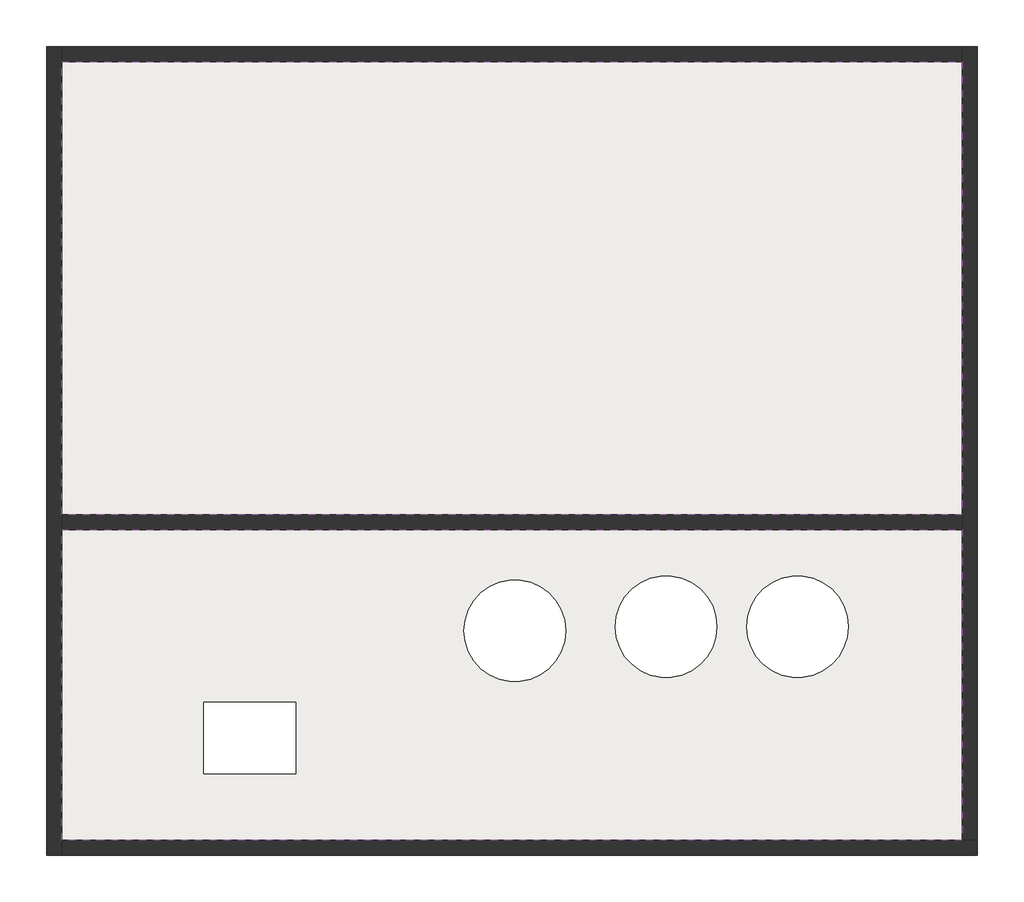
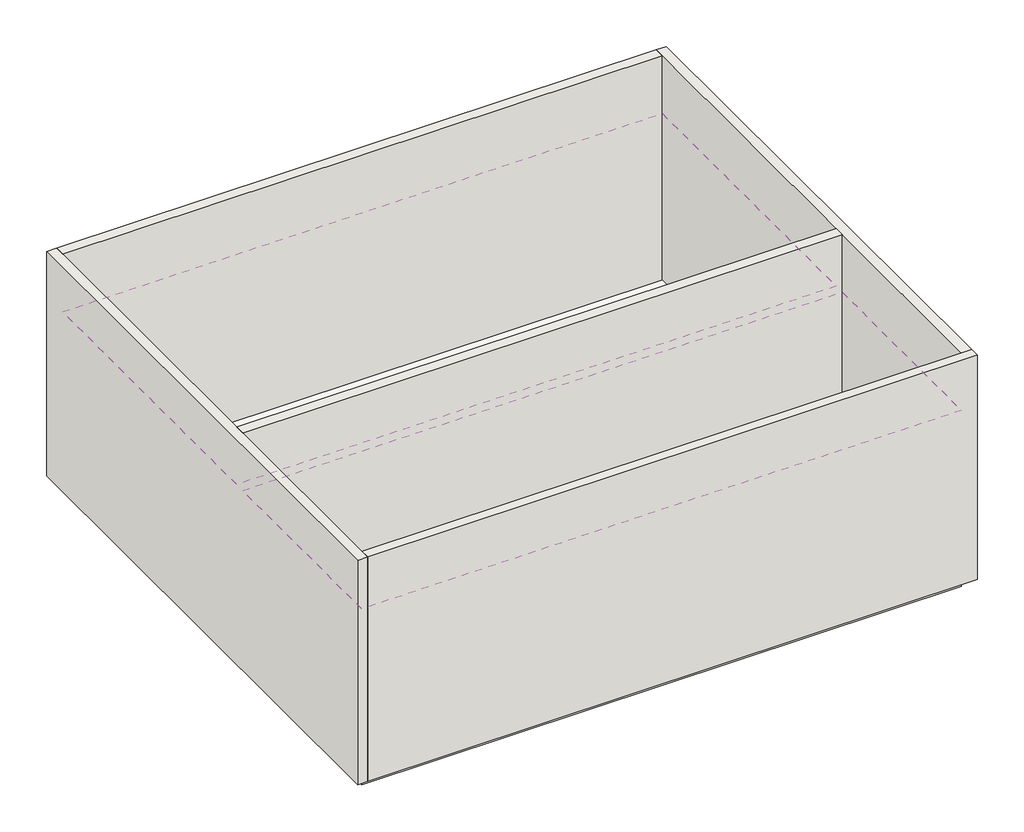
# One storey: 5 walls, 2 coverings, 1 slab.
"""IFC4 building model written with IfcOpenShell, lengths in millimetres."""

from ifc_helpers import new_model, si_unit, point, frame, frame_2d, origin, place, context, project, spatial, polyline, circle_curve, trimmed, segment, composite_curve, outline, extrude, faceted_brep, element, save

model = new_model("IFC4")

# Units and contexts
model_context = context("Model", 3, world=origin())
ifc_project = project(units=[si_unit("LENGTHUNIT", "METRE", prefix="MILLI")], contexts=[model_context])

# Site, building, storey
site = spatial("IfcSite", under=ifc_project)
building = spatial("IfcBuilding", under=site)
storey = spatial("IfcBuildingStorey", under=building, Name="レベル 2", Elevation=4000.0)

# Coverings
placement = place(None, origin())
element("IfcCovering", 1, ObjectType="グリッド 600x600mm", at=placement, inside=storey, context=model_context, shape_type="SweptSolid", body=[
    extrude(outline(polyline([(-1039.1497645, -1548.6940898), (-9889.1497645, -1548.6940898), (-9889.1497645, 2901.3059102), (-1039.1497645, 2901.3059102), (-1039.1497645, -1548.6940898)])), frame((0.0, 0.0, 6600.0), z_axis=(0.0, 0.0, 1.0), x_axis=(1.0, 0.0, 0.0)), (0.0, 0.0, 1.0), 52.0),
])
element("IfcCovering", 2, ObjectType="グリッド 600x600mm", at=placement, inside=storey, context=model_context, shape_type="SweptSolid", body=[
    extrude(outline(polyline([(-1039.1497645, -1698.6940898), (-1039.1497645, -4748.6940898), (-9889.1497645, -4748.6940898), (-9889.1497645, -1698.6940898), (-1039.1497645, -1698.6940898)]), holes=[polyline([(-7591.6429011, -4094.9873293), (-7591.6429011, -3394.9873293), (-8491.6429011, -3394.9873293), (-8491.6429011, -4094.9873293), (-7591.6429011, -4094.9873293)]), composite_curve([segment(trimmed(circle_curve(frame_2d((-5436.6640818, -2690.8635378)), 500.0), [point((-5436.6640818, -2190.8635378))], [point((-5436.6640818, -3190.8635378))], True, "CARTESIAN"), True, "CONTINUOUS"), segment(trimmed(circle_curve(frame_2d((-5436.6640818, -2690.8635378)), 500.0), [point((-5436.6640818, -3190.8635378))], [point((-5436.6640818, -2190.8635378))], True, "CARTESIAN"), True, "CONTINUOUS")], self_intersect=False), composite_curve([segment(trimmed(circle_curve(frame_2d((-3949.3788791, -2650.2471348)), 500.0), [point((-3949.3788791, -2150.2471348))], [point((-3949.3788791, -3150.2471348))], True, "CARTESIAN"), True, "CONTINUOUS"), segment(trimmed(circle_curve(frame_2d((-3949.3788791, -2650.2471348)), 500.0), [point((-3949.3788791, -3150.2471348))], [point((-3949.3788791, -2150.2471348))], True, "CARTESIAN"), True, "CONTINUOUS")], self_intersect=False), composite_curve([segment(trimmed(circle_curve(frame_2d((-2657.8130196, -2650.2471348)), 500.0), [point((-2657.8130196, -2150.2471348))], [point((-2657.8130196, -3150.2471348))], True, "CARTESIAN"), True, "CONTINUOUS"), segment(trimmed(circle_curve(frame_2d((-2657.8130196, -2650.2471348)), 500.0), [point((-2657.8130196, -3150.2471348))], [point((-2657.8130196, -2150.2471348))], True, "CARTESIAN"), True, "CONTINUOUS")], self_intersect=False)]), frame((0.0, 0.0, 6600.0), z_axis=(0.0, 0.0, 1.0), x_axis=(1.0, 0.0, 0.0)), (0.0, 0.0, 1.0), 52.0),
])

# Slab
element("IfcSlab", 3, ObjectType="一般 150 mm", at=placement, inside=storey, context=model_context, shape_type="SweptSolid", body=[
    extrude(outline(polyline([(-1039.1497645, 2901.3059102), (-1039.1497645, -4748.6940898), (-9889.1497645, -4748.6940898), (-9889.1497645, 2901.3059102), (-1039.1497645, 2901.3059102)]), holes=[polyline([(-7591.6429011, -3394.9873293), (-8491.6429011, -3394.9873293), (-8491.6429011, -4094.9873293), (-7591.6429011, -4094.9873293), (-7591.6429011, -3394.9873293)]), composite_curve([segment(trimmed(circle_curve(frame_2d((-5436.6640818, -2690.8635378)), 500.0), [point((-4936.6640818, -2690.8635378))], [point((-5936.6640818, -2690.8635378))], True, "CARTESIAN"), True, "CONTINUOUS"), segment(trimmed(circle_curve(frame_2d((-5436.6640818, -2690.8635378)), 500.0), [point((-5936.6640818, -2690.8635378))], [point((-4936.6640818, -2690.8635378))], True, "CARTESIAN"), True, "CONTINUOUS")], self_intersect=False), composite_curve([segment(trimmed(circle_curve(frame_2d((-3949.3788791, -2650.2471348)), 500.0), [point((-3449.3788791, -2650.2471348))], [point((-4449.3788791, -2650.2471348))], True, "CARTESIAN"), True, "CONTINUOUS"), segment(trimmed(circle_curve(frame_2d((-3949.3788791, -2650.2471348)), 500.0), [point((-4449.3788791, -2650.2471348))], [point((-3449.3788791, -2650.2471348))], True, "CARTESIAN"), True, "CONTINUOUS")], self_intersect=False), composite_curve([segment(trimmed(circle_curve(frame_2d((-2657.8130196, -2650.2471348)), 500.0), [point((-2157.8130196, -2650.2471348))], [point((-3157.8130196, -2650.2471348))], True, "CARTESIAN"), True, "CONTINUOUS"), segment(trimmed(circle_curve(frame_2d((-2657.8130196, -2650.2471348)), 500.0), [point((-3157.8130196, -2650.2471348))], [point((-2157.8130196, -2650.2471348))], True, "CARTESIAN"), True, "CONTINUOUS")], self_intersect=False)]), frame((0.0, 0.0, 3850.0), z_axis=(0.0, 0.0, 1.0), x_axis=(1.0, 0.0, 0.0)), (0.0, 0.0, 1.0), 150.0),
])

# Walls
element("IfcWall", 4, ObjectType="標準-150mm", at=placement, inside=storey, context=model_context, shape_type="Brep", body=[
    faceted_brep([(-10039.1497645, 3051.3059102, 4000.0), (-10039.1497645, -4898.6940898, 4000.0), (-10039.1497645, -4898.6940898, 7500.0), (-10039.1497645, 3051.3059102, 7500.0), (-9889.1497645, 3051.3059102, 4000.0), (-9889.1497645, 3051.3059102, 7500.0), (-9889.1497645, 2901.3059102, 7500.0), (-9889.1497645, -1548.6940898, 7500.0), (-9889.1497645, -1698.6940898, 7500.0), (-9889.1497645, -4748.6940898, 7500.0), (-9889.1497645, -4898.6940898, 7500.0), (-9889.1497645, -4898.6940898, 4000.0), (-9889.1497645, -4748.6940898, 4000.0), (-9889.1497645, -1698.6940898, 4000.0), (-9889.1497645, -1548.6940898, 4000.0), (-9889.1497645, 2901.3059102, 4000.0)], [[[0, 1, 2, 3]], [[4, 5, 6, 7, 8, 9, 10, 11, 12, 13, 14, 15]], [[1, 0, 4, 15, 14, 13, 12, 11]], [[3, 2, 10, 9, 8, 7, 6, 5]], [[0, 3, 5, 4]], [[2, 1, 11, 10]]]),
])
element("IfcWall", 5, ObjectType="標準-150mm", at=placement, inside=storey, context=model_context, shape_type="SweptSolid", body=[
    extrude(outline(polyline([(-1039.1497645, -1698.6940898), (-9889.1497645, -1698.6940898), (-9889.1497645, -1548.6940898), (-1039.1497645, -1548.6940898), (-1039.1497645, -1698.6940898)])), frame((0.0, 0.0, 4000.0), z_axis=(0.0, 0.0, 1.0), x_axis=(1.0, 0.0, 0.0)), (0.0, 0.0, 1.0), 3500.0),
])
element("IfcWall", 6, ObjectType="標準-150mm", at=placement, inside=storey, context=model_context, shape_type="Brep", body=[
    faceted_brep([(-889.1497645, -4748.6940898, 4000.0), (-889.1497645, 3051.3059102, 4000.0), (-889.1497645, 3051.3059102, 7500.0), (-889.1497645, -4748.6940898, 7500.0), (-1039.1497645, -4748.6940898, 4000.0), (-1039.1497645, -4748.6940898, 7500.0), (-1039.1497645, -1698.6940898, 7500.0), (-1039.1497645, -1548.6940898, 7500.0), (-1039.1497645, 2901.3059102, 7500.0), (-1039.1497645, 3051.3059102, 7500.0), (-1039.1497645, 3051.3059102, 4000.0), (-1039.1497645, 2901.3059102, 4000.0), (-1039.1497645, -1548.6940898, 4000.0), (-1039.1497645, -1698.6940898, 4000.0)], [[[0, 1, 2, 3]], [[4, 5, 6, 7, 8, 9, 10, 11, 12, 13]], [[1, 0, 4, 13, 12, 11, 10]], [[3, 2, 9, 8, 7, 6, 5]], [[2, 1, 10, 9]], [[0, 3, 5, 4]]]),
])
element("IfcWall", 7, ObjectType="標準-150mm", at=placement, inside=storey, context=model_context, shape_type="SweptSolid", body=[
    extrude(outline(polyline([(-9889.1497645, 3051.3059102), (-1039.1497645, 3051.3059102), (-1039.1497645, 2901.3059102), (-9889.1497645, 2901.3059102), (-9889.1497645, 3051.3059102)])), frame((0.0, 0.0, 4000.0), z_axis=(0.0, 0.0, 1.0), x_axis=(1.0, 0.0, 0.0)), (0.0, 0.0, 1.0), 3500.0),
])
element("IfcWall", 8, ObjectType="標準-150mm", at=placement, inside=storey, context=model_context, shape_type="Brep", body=[
    faceted_brep([(-9889.1497645, -4898.6940898, 4000.0), (-889.1497645, -4898.6940898, 4000.0), (-889.1497645, -4898.6940898, 7500.0), (-9889.1497645, -4898.6940898, 7500.0), (-9889.1497645, -4748.6940898, 4000.0), (-9889.1497645, -4748.6940898, 7500.0), (-1039.1497645, -4748.6940898, 7500.0), (-889.1497645, -4748.6940898, 7500.0), (-889.1497645, -4748.6940898, 4000.0), (-1039.1497645, -4748.6940898, 4000.0)], [[[0, 1, 2, 3]], [[4, 5, 6, 7, 8, 9]], [[1, 0, 4, 9, 8]], [[3, 2, 7, 6, 5]], [[0, 3, 5, 4]], [[2, 1, 8, 7]]]),
])

save(model, "model.ifc")

# Revit data of these elements
# Type "グリッド 600x600mm"
#   built-in parameter 1002203 = 1 (stored number, unit not read)
#   built-in parameter 1002202 = 1 (stored number, unit not read)
#   Layers, outside or top first: 36 mm no material (function 1); 16 mm "天井タイル 600 x 600" (function 5)
# Type "一般 150 mm"
#   Function = 0
#   Layers, outside or top first: 150 mm no material (function 1)
# Type "標準-150mm"
#   Layers, outside or top first: 150 mm no material (function 1)
# Elements 1, 2 (IfcCovering, "グリッド 600x600mm")
#   Height Offset From Level = 2600 mm
#   Phase Created = 新しい建設
#   Materials on its faces: "天井タイル 600 x 600"
# Element 3 (IfcSlab, "一般 150 mm")
#   Height Offset From Level = 0 mm
#   Phase Created = 新しい建設
# Elements 4, 5, 6, 7, 8 (IfcWall, "標準-150mm")
#   Top Offset = 3500 mm
#   Base Offset = 0 mm
#   wall height = 3500 mm
#   Phase Created = 新しい建設
#   Base Constraint = レベル 2
#   Top Constraint = レベル 2
#   Materials on its faces: "既定の壁"
# Materials
#   "天井タイル 600 x 600": class "一般", colour RGB 235 235 235, transparency 0, Description = "吸音天井タイル", Cost = 0
#   "既定の壁": class "その他", colour RGB 127 127 127, transparency 0, Cost = 0
